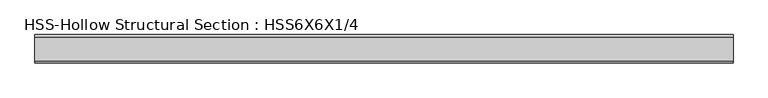
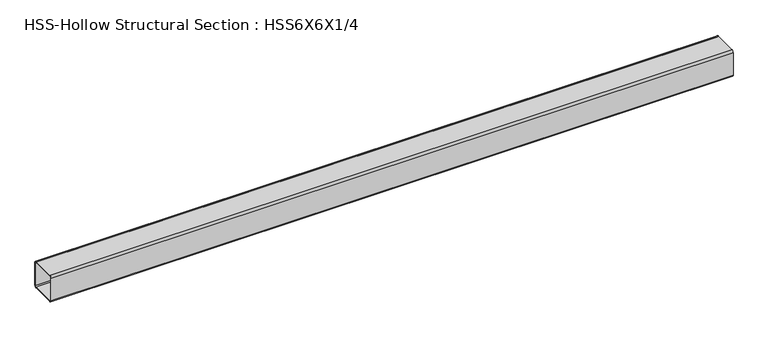
"""IFC4 building model written with IfcOpenShell, lengths in millimetres: beam geometry, HSS-Hollow Structural Section : HSS6X6X1/4."""

from ifc_helpers import new_model, si_unit, point, frame, frame_2d, origin, place, context, project, spatial, polyline, circle_curve, trimmed, segment, composite_curve, outline, extrude, source, transform, mapped, element, save


def hss_hollow_structural_section_hss6x6x1_4_3816dc0f(model_context):
    return source(origin(), model_context, "Body", "SweptSolid", [
        extrude(outline(composite_curve([segment(polyline([(76.2, 64.3636), (76.2, -64.3636)]), True, "CONTINUOUS"), segment(trimmed(circle_curve(frame_2d((64.3636, -64.3636)), 11.8364), [point((76.2, -64.3636))], [point((64.3636, -76.2))], False, "CARTESIAN"), True, "CONTINUOUS"), segment(polyline([(64.3636, -76.2), (-64.3636, -76.2)]), True, "CONTINUOUS"), segment(trimmed(circle_curve(frame_2d((-64.3636, -64.3636)), 11.8364), [point((-64.3636, -76.2))], [point((-76.2, -64.3636))], False, "CARTESIAN"), True, "CONTINUOUS"), segment(polyline([(-76.2, -64.3636), (-76.2, 64.3636)]), True, "CONTINUOUS"), segment(trimmed(circle_curve(frame_2d((-64.3636, 64.3636)), 11.8364), [point((-76.2, 64.3636))], [point((-64.3636, 76.2))], False, "CARTESIAN"), True, "CONTINUOUS"), segment(polyline([(-64.3636, 76.2), (64.3636, 76.2)]), True, "CONTINUOUS"), segment(trimmed(circle_curve(frame_2d((64.3636, 64.3636)), 11.8364), [point((64.3636, 76.2))], [point((76.2, 64.3636))], False, "CARTESIAN"), True, "CONTINUOUS")], self_intersect=False), holes=[composite_curve([segment(trimmed(circle_curve(frame_2d((-64.3636, 64.3636)), 5.9182), [point((-64.3636, 70.2818))], [point((-70.2818, 64.3636))], True, "CARTESIAN"), True, "CONTINUOUS"), segment(polyline([(-70.2818, 64.3636), (-70.2818, -64.3636)]), True, "CONTINUOUS"), segment(trimmed(circle_curve(frame_2d((-64.3636, -64.3636)), 5.9182), [point((-70.2818, -64.3636))], [point((-64.3636, -70.2818))], True, "CARTESIAN"), True, "CONTINUOUS"), segment(polyline([(-64.3636, -70.2818), (64.3636, -70.2818)]), True, "CONTINUOUS"), segment(trimmed(circle_curve(frame_2d((64.3636, -64.3636)), 5.9182), [point((64.3636, -70.2818))], [point((70.2818, -64.3636))], True, "CARTESIAN"), True, "CONTINUOUS"), segment(polyline([(70.2818, -64.3636), (70.2818, 64.3636)]), True, "CONTINUOUS"), segment(trimmed(circle_curve(frame_2d((64.3636, 64.3636)), 5.9182), [point((70.2818, 64.3636))], [point((64.3636, 70.2818))], True, "CARTESIAN"), True, "CONTINUOUS"), segment(polyline([(64.3636, 70.2818), (-64.3636, 70.2818)]), True, "CONTINUOUS")], self_intersect=False)]), frame((-1866.9, 0.0, 0.0), z_axis=(1.0, 0.0, 0.0), x_axis=(0.0, 1.0, 0.0)), (0.0, 0.0, 1.0), 3733.8),
    ])


if __name__ == "__main__":
    model = new_model("IFC4")
    model_context = context("Model", 3, world=origin())
    ifc_project = project(units=[si_unit("LENGTHUNIT", "METRE", prefix="MILLI")], contexts=[model_context])
    site = spatial("IfcSite", under=ifc_project)
    building = spatial("IfcBuilding", under=site)
    placement = place(None, origin())
    hss_hollow_structural_section_hss6x6x1_4_shape = hss_hollow_structural_section_hss6x6x1_4_3816dc0f(model_context)
    element("IfcBeam", 1, ObjectType="HSS-Hollow Structural Section : HSS6X6X1/4", at=placement, inside=building, context=model_context, shape_type="MappedRepresentation", body=[
        mapped(hss_hollow_structural_section_hss6x6x1_4_shape, transform((0.0, 0.0, 0.0), x_axis=(1.0, 0.0, 0.0), y_axis=(0.0, 1.0, 0.0), z_axis=(0.0, 0.0, 1.0))),
    ])
    save(model, "model.ifc")

# Revit data of these elements
# Type "HSS-Hollow Structural Section : HSS6X6X1/4"
#   Assembly Code = "B10"
#   Shape = "Square"
#   W = 19
#   Ht = 0' - 6"
#   Length [instance default] = 5' - 0"
#   b = 0' - 6"
#   kr = 0' - 0.466"
#   t = 0' - 0.233"
#   A = 0.0363889 SF
#   Structural Material [instance default] = Steel ASTM A500, Grade B, Rectangular and Square
# Element 1 (IfcBeam, "HSS-Hollow Structural Section : HSS6X6X1/4")
#   Materials on its faces: "Steel ASTM A500, Grade B, Rectangular and Square"
# Materials
#   "Steel ASTM A500, Grade B, Rectangular and Square": class "Metal", colour RGB 199 199 199, transparency 0, Description = "Carbon steel", Cost = 0
